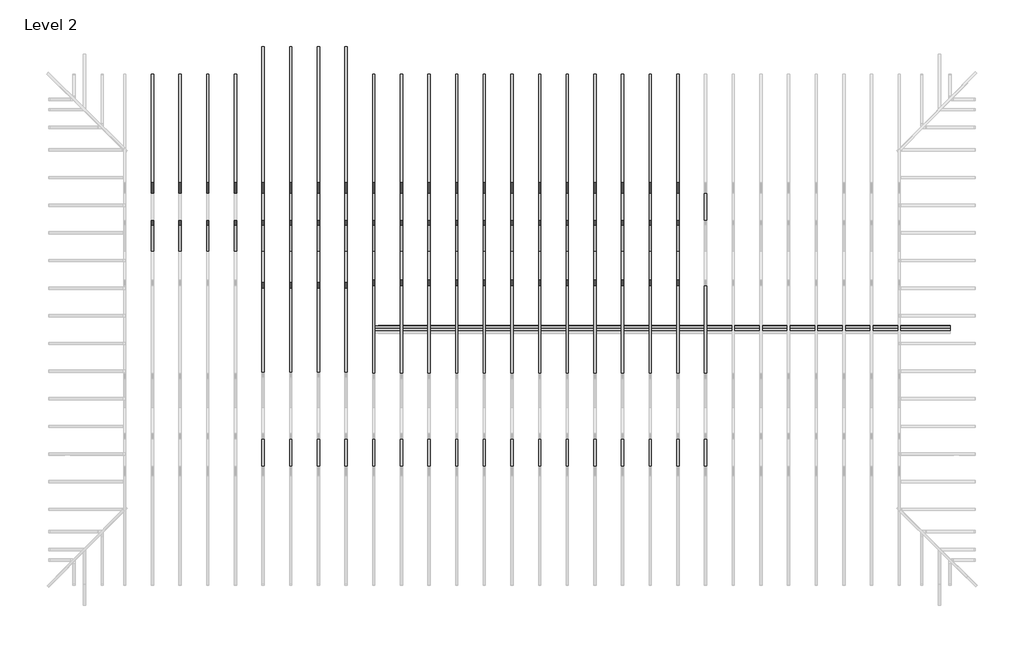
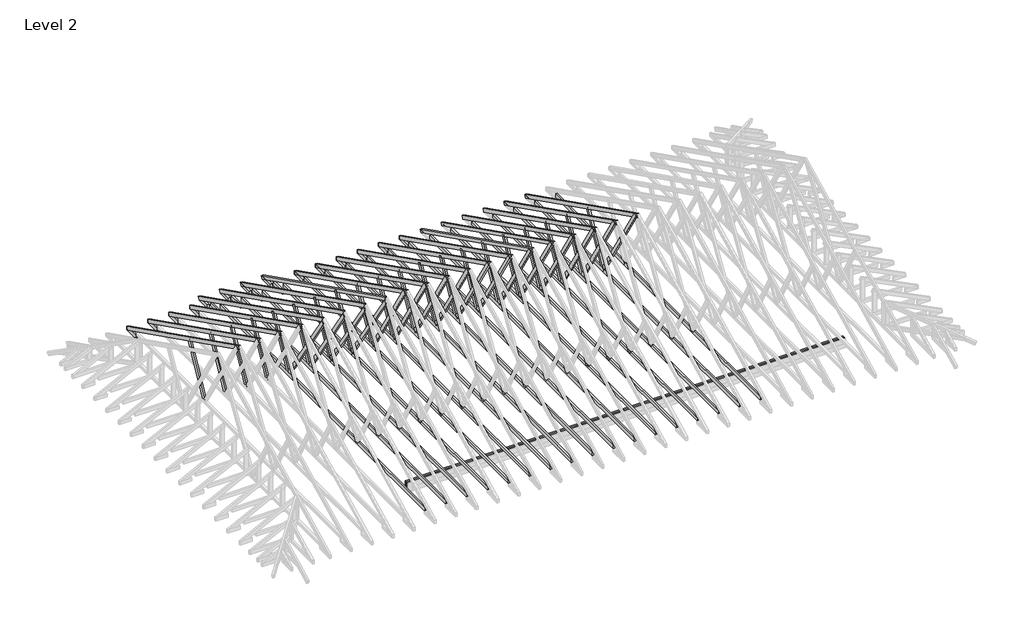
# One storey, part 4 of 5: 97 beams.
"""IFC4 building model written with IfcOpenShell, lengths in millimetres."""

import ifcopenshell
import ifcopenshell.guid

model = None  # the IFC model being written
_history = None  # IfcOwnerHistory: only IFC2X3 demands one
_inside = {}  # id of a spatial element -> (the spatial element, [elements in it])
_under = {}  # id of a project, library or spatial element -> (it, [spatial elements below it])
_declared = {}  # id of a project -> (the project, [libraries it declares])
_typed = {}  # id of a type object -> (the type object, [elements of that type])
_made_of = {}  # id of a material, layer set ... -> (it, [elements and type objects made of it])


def new_model(schema):
    """Start an empty IFC model of exactly this schema.

    Asked for "IFC4X3", IfcOpenShell would pick the latest addendum, in which some entities
    have other attributes; the version numbers below select the first issue.
    IFC2X3 requires an IfcOwnerHistory on every rooted entity: one is made here for all.
    """
    global model, _history
    if schema == "IFC4X3":
        model = ifcopenshell.file(schema_version=(4, 3, 0, 0))
    else:
        model = ifcopenshell.file(schema=schema)
    _inside.clear()
    _under.clear()
    _declared.clear()
    _typed.clear()
    _made_of.clear()
    _history = None
    if model.schema == "IFC2X3":
        org = make("IfcOrganization", Name="unknown")
        user = make(
            "IfcPersonAndOrganization",
            ThePerson=make("IfcPerson", FamilyName="unknown"),
            TheOrganization=org,
        )
        app = make(
            "IfcApplication",
            ApplicationDeveloper=org,
            Version="unknown",
            ApplicationFullName="unknown",
            ApplicationIdentifier="unknown",
        )
        _history = make(
            "IfcOwnerHistory",
            OwningUser=user,
            OwningApplication=app,
            ChangeAction="ADDED",
            CreationDate=0,
        )
    return model


def make(cls, **values):
    """One entity of the class cls with the attributes given. An attribute that is None is left unset."""
    return model.create_entity(
        cls, **{name: value for name, value in values.items() if value is not None}
    )


def rooted(cls, **values):
    """An entity with a GlobalId (a new one), such as an element, a storey or a relation."""
    return make(cls, GlobalId=ifcopenshell.guid.new(), OwnerHistory=_history, **values)


def si_unit(unit_type, name, prefix=None):
    """IfcSIUnit, for example si_unit("LENGTHUNIT", "METRE", prefix="MILLI")."""
    return make("IfcSIUnit", UnitType=unit_type, Prefix=prefix, Name=name)


def assignment(units):
    """IfcUnitAssignment: the units of a project."""
    return None if units is None else make("IfcUnitAssignment", Units=units)


def point(xyz):
    """IfcCartesianPoint."""
    return None if xyz is None else make("IfcCartesianPoint", Coordinates=xyz)


def direction(xyz):
    """IfcDirection."""
    return None if xyz is None else make("IfcDirection", DirectionRatios=xyz)


def frame(location, z_axis=None, x_axis=None):
    """IfcAxis2Placement3D, a coordinate frame: its origin and axes. An axis left out is left unset."""
    return make(
        "IfcAxis2Placement3D",
        Location=point(location),
        Axis=direction(z_axis),
        RefDirection=direction(x_axis),
    )


def origin():
    """The frame at (0, 0, 0) with its axes left unset."""
    return frame((0.0, 0.0, 0.0))


def place(relative_to, where):
    """IfcLocalPlacement: puts the frame where relative to a parent placement (None: the world)."""
    return make(
        "IfcLocalPlacement", PlacementRelTo=relative_to, RelativePlacement=where
    )


def context(
    kind, dimensions, precision=None, world=None, true_north=None, identifier=None
):
    """IfcGeometricRepresentationContext, for example the 3D "Model" context."""
    return make(
        "IfcGeometricRepresentationContext",
        ContextIdentifier=identifier,
        ContextType=kind,
        CoordinateSpaceDimension=dimensions,
        Precision=precision,
        WorldCoordinateSystem=world,
        TrueNorth=true_north,
    )


def project(units=None, contexts=None):
    """IfcProject with its units and contexts."""
    return rooted(
        "IfcProject",
        Name="project",
        RepresentationContexts=contexts,
        UnitsInContext=assignment(units),
    )


def spatial(cls, under=None, at=None, **own):
    """A site, building, storey or space (cls), placed at a placement, below another one or the project."""
    s = rooted(cls, ObjectPlacement=at, **own)
    if under is not None:
        _under.setdefault(under.id(), (under, []))[1].append(s)
    return s


def polyline(points):
    """IfcPolyline through the points."""
    return make("IfcPolyline", Points=[point(p) for p in points])


def outline(outer, holes=None, kind="AREA"):
    """IfcArbitraryClosedProfileDef: a profile drawn as a closed curve; with holes, ...WithVoids."""
    if holes is None:
        return make("IfcArbitraryClosedProfileDef", ProfileType=kind, OuterCurve=outer)
    return make(
        "IfcArbitraryProfileDefWithVoids",
        ProfileType=kind,
        OuterCurve=outer,
        InnerCurves=holes,
    )


def extrude(swept, where, along, depth):
    """IfcExtrudedAreaSolid: the profile swept, set in the frame where, extruded along a direction by depth."""
    return make(
        "IfcExtrudedAreaSolid",
        SweptArea=swept,
        Position=where,
        ExtrudedDirection=direction(along),
        Depth=depth,
    )


def shape(context_of_items, identifier, shape_type, items):
    """IfcShapeRepresentation: the items that make up one representation, for example the "Body"."""
    return make(
        "IfcShapeRepresentation",
        ContextOfItems=context_of_items,
        RepresentationIdentifier=identifier,
        RepresentationType=shape_type,
        Items=items,
    )


def source(mapping_origin, context_of_items, identifier, shape_type, items):
    """IfcRepresentationMap: a shape defined once, which mapped items show again and again."""
    return make(
        "IfcRepresentationMap",
        MappingOrigin=mapping_origin,
        MappedRepresentation=shape(context_of_items, identifier, shape_type, items),
    )


def transform(
    local_origin,
    x_axis=None,
    y_axis=None,
    z_axis=None,
    scale=None,
    scale2=None,
    scale3=None,
    uniform=True,
):
    """IfcCartesianTransformationOperator3D, or its non-uniform kind. x_axis, y_axis, z_axis: its Axis1, 2, 3."""
    if uniform:
        return make(
            "IfcCartesianTransformationOperator3D",
            Axis1=direction(x_axis),
            Axis2=direction(y_axis),
            LocalOrigin=point(local_origin),
            Scale=scale,
            Axis3=direction(z_axis),
        )
    return make(
        "IfcCartesianTransformationOperator3DnonUniform",
        Axis1=direction(x_axis),
        Axis2=direction(y_axis),
        LocalOrigin=point(local_origin),
        Scale=scale,
        Axis3=direction(z_axis),
        Scale2=scale2,
        Scale3=scale3,
    )


def mapped(mapping_source, mapping_target):
    """IfcMappedItem: shows the shape of a source again, moved by a transform."""
    return make(
        "IfcMappedItem", MappingSource=mapping_source, MappingTarget=mapping_target
    )


def made_of(thing, what):
    """Note that an element or type object is made of a material, layer set ...; save() writes the relation."""
    if what is not None:
        _made_of.setdefault(what.id(), (what, []))[1].append(thing)
    return thing


def element(
    cls,
    number,
    at=None,
    inside=None,
    cuts=None,
    type_object=None,
    material=None,
    context=None,
    identifier="Body",
    shape_type=None,
    held_by="IfcProductDefinitionShape",
    body=None,
    shapes=None,
    **own,
):
    """One element of the class cls, such as IfcWall. Its Tag is "e" and its number.

    at: its placement. inside: the storey or other place that contains it. cuts: it is an
    opening in that element (IfcRelVoidsElement). A single representation is given by context,
    identifier, shape_type and body (its items); several are given by shapes. held_by: the class
    of the entity that holds the representations. save() writes the other relations.
    """
    e = rooted(cls, Tag="e%d" % number, ObjectPlacement=at, **own)
    if body is not None:
        shapes = [shape(context, identifier, shape_type, body)]
    if shapes is not None:
        e.Representation = make(held_by, Representations=shapes)
    if inside is not None:
        _inside.setdefault(inside.id(), (inside, []))[1].append(e)
    if cuts is not None:
        rooted(
            "IfcRelVoidsElement", RelatingBuildingElement=cuts, RelatedOpeningElement=e
        )
    if type_object is not None:
        _typed.setdefault(type_object.id(), (type_object, []))[1].append(e)
    return made_of(e, material)


def aggregate(whole, parts):
    """IfcRelAggregates: a whole, such as a stair, and the parts it consists of."""
    return rooted("IfcRelAggregates", RelatingObject=whole, RelatedObjects=parts)


def save(model, path):
    """Write the relations noted so far, then the file.

    IfcRelAggregates (storeys below a building ...), IfcRelContainedInSpatialStructure (elements
    in a storey), IfcRelDefinesByType, IfcRelAssociatesMaterial and IfcRelDeclares: one each for
    every whole, place, type object, material and project.
    """
    for whole, parts in _under.values():
        aggregate(whole, parts)
    for where, things in _inside.values():
        rooted(
            "IfcRelContainedInSpatialStructure",
            RelatedElements=things,
            RelatingStructure=where,
        )
    for kind, things in _typed.values():
        rooted("IfcRelDefinesByType", RelatedObjects=things, RelatingType=kind)
    for what, things in _made_of.values():
        rooted("IfcRelAssociatesMaterial", RelatedObjects=things, RelatingMaterial=what)
    for by, libraries in _declared.values():
        rooted("IfcRelDeclares", RelatingContext=by, RelatedDefinitions=libraries)
    model.write(path)


def beam_b78a0881(model_context):
    return source(origin(), model_context, "Body", "SweptSolid", [
        extrude(outline(polyline([(228.6, 25.4), (228.6, -25.4), (-228.6, -25.4), (-228.6, 25.4), (228.6, 25.4)])), frame((0.0, 0.0, -50.8), z_axis=(0.0, 0.0, 1.0), x_axis=(1.0, 0.0, 0.0)), (0.0, 0.0, 1.0), 101.6),
    ])


def beam_90eea034(model_context):
    return source(origin(), model_context, "Body", "SweptSolid", [
        extrude(outline(polyline([(821.193698, 25.4), (821.193698, -25.4), (-819.5010489, -25.4), (-819.5010489, 25.4), (821.193698, 25.4)])), frame((0.0, 0.0, -50.8), z_axis=(0.0, 0.0, 1.0), x_axis=(1.0, 0.0, 0.0)), (0.0, 0.0, 1.0), 101.6),
    ])


def beam_a4242642(model_context):
    return source(origin(), model_context, "Body", "SweptSolid", [
        extrude(outline(polyline([(5145.3336481, 25.4), (5145.3336481, -25.4), (-5145.3336481, -25.4), (-5145.3336481, 25.4), (5145.3336481, 25.4)])), frame((0.0, 0.0, -50.8), z_axis=(0.0, 0.0, 1.0), x_axis=(1.0, 0.0, 0.0)), (0.0, 0.0, 1.0), 101.6),
    ])


def beam_fc8bf4ae(model_context):
    return source(origin(), model_context, "Body", "SweptSolid", [
        extrude(outline(polyline([(1562.6646551, 25.4), (1562.6646551, -25.4), (-1550.1468127, -25.4), (-1550.1468127, 25.4), (1562.6646551, 25.4)])), frame((0.0, 0.0, -50.8), z_axis=(0.0, 0.0, 1.0), x_axis=(1.0, 0.0, 0.0)), (0.0, 0.0, 1.0), 101.6),
    ])


def beam_2924e986(model_context):
    return source(origin(), model_context, "Body", "SweptSolid", [
        extrude(outline(polyline([(228.5999994, 25.4), (228.5999994, -25.4), (-179.8629717, -25.4), (-179.8629717, 25.4), (228.5999994, 25.4)])), frame((0.0, 0.0, -50.8), z_axis=(0.0, 0.0, 1.0), x_axis=(1.0, 0.0, 0.0)), (0.0, 0.0, 1.0), 101.6),
    ])


def beam_189f326c(model_context):
    return source(origin(), model_context, "Body", "SweptSolid", [
        extrude(outline(polyline([(1574.4380265, 25.4), (1574.4380265, -25.4), (-1601.4606477, -25.4), (-1601.4606477, 25.4), (1574.4380265, 25.4)])), frame((0.0, 0.0, -50.8), z_axis=(0.0, 0.0, 1.0), x_axis=(1.0, 0.0, 0.0)), (0.0, 0.0, 1.0), 101.6),
    ])


def beam_af7bd0b6(model_context):
    return source(origin(), model_context, "Body", "SweptSolid", [
        extrude(outline(polyline([(228.6, 25.4), (228.6, -25.4), (-179.8629717, -25.4), (-179.8629717, 25.4), (228.6, 25.4)])), frame((0.0, 0.0, -50.8), z_axis=(0.0, 0.0, 1.0), x_axis=(1.0, 0.0, 0.0)), (0.0, 0.0, 1.0), 101.6),
    ])


def beam_bcf194da(model_context):
    return source(origin(), model_context, "Body", "SweptSolid", [
        extrude(outline(polyline([(6302.375, 25.4), (6302.375, -25.4), (-6429.375, -25.4), (-6429.375, 25.4), (6302.375, 25.4)])), frame((0.0, 0.0, -127.0), z_axis=(0.0, 0.0, 1.0), x_axis=(1.0, 0.0, 0.0)), (0.0, 0.0, 1.0), 254.0),
    ])


def beam_af2566d3(model_context):
    return source(origin(), model_context, "Body", "SweptSolid", [
        extrude(outline(polyline([(6458.3020508, 5.55625), (6458.3020508, -5.55625), (-6159.1479492, -5.55625), (-6159.1479492, 5.55625), (6458.3020508, 5.55625)])), frame((0.0, 0.0, -63.5), z_axis=(0.0, 0.0, 1.0), x_axis=(1.0, 0.0, 0.0)), (0.0, 0.0, 1.0), 127.0),
    ])


model = new_model("IFC4")

# Units and contexts
model_context = context("Model", 3, world=origin())
ifc_project = project(units=[si_unit("LENGTHUNIT", "METRE", prefix="MILLI")], contexts=[model_context])

# Site, building, storey
site = spatial("IfcSite", under=ifc_project)
building = spatial("IfcBuilding", under=site)
storey = spatial("IfcBuildingStorey", under=building, Name="Level 2", Elevation=2768.6)

# Beams
placement = place(None, origin())
element("IfcBeam", 1, ObjectType="Dimension Lumber : BLDG 6241 2X4\" TRUSS MEMBER", at=placement, inside=storey, context=model_context, shape_type="SweptSolid", body=[
    extrude(outline(polyline([(0.0, -50.8), (0.0, 0.0), (6948.260151, 0.0), (6948.260151, -50.8), (0.0, -50.8)])), frame((-13559.414829, 10.7781069, 5482.082899), z_axis=(0.0, 0.4472135954999579, 0.894427190999916), x_axis=(0.0, 0.894427190999916, -0.4472135954999579)), (0.0, 0.0, 1.0), 101.6),
])
element("IfcBeam", 2, ObjectType="Dimension Lumber : BLDG 6241 2X4\" TRUSS MEMBER", at=placement, inside=storey, context=model_context, shape_type="SweptSolid", body=[
    extrude(outline(polyline([(0.0, -50.8), (0.0, 0.0), (6948.260151, 0.0), (6948.260151, -50.8), (0.0, -50.8)])), frame((-12949.814829, 10.7781069, 5482.082899), z_axis=(0.0, 0.44721359549995804, 0.894427190999916), x_axis=(0.0, 0.894427190999916, -0.44721359549995804)), (0.0, 0.0, 1.0), 101.6),
])
element("IfcBeam", 3, ObjectType="Dimension Lumber : BLDG 6241 2X4\" TRUSS MEMBER", at=placement, inside=storey, context=model_context, shape_type="SweptSolid", body=[
    extrude(outline(polyline([(0.0, -50.8), (0.0, 0.0), (6948.260151, 0.0), (6948.260151, -50.8), (0.0, -50.8)])), frame((-12340.214829, 10.7781069, 5482.082899), z_axis=(0.0, 0.44721359549995804, 0.894427190999916), x_axis=(0.0, 0.894427190999916, -0.44721359549995804)), (0.0, 0.0, 1.0), 101.6),
])
element("IfcBeam", 4, ObjectType="Dimension Lumber : BLDG 6241 2X4\" TRUSS MEMBER", at=placement, inside=storey, context=model_context, shape_type="SweptSolid", body=[
    extrude(outline(polyline([(0.0, -50.8), (0.0, 0.0), (6948.260151, 0.0), (6948.260151, -50.8), (0.0, -50.8)])), frame((-11730.614829, 10.7781069, 5482.082899), z_axis=(0.0, 0.44721359549995804, 0.894427190999916), x_axis=(0.0, 0.894427190999916, -0.44721359549995804)), (0.0, 0.0, 1.0), 101.6),
])
element("IfcBeam", 5, ObjectType="Dimension Lumber : BLDG 6241 2X4\" TRUSS MEMBER", at=placement, inside=storey, context=model_context, shape_type="SweptSolid", body=[
    extrude(outline(polyline([(0.0, -50.8), (0.0, 0.0), (6302.2496334, 0.0), (6302.2496334, -50.8), (0.0, -50.8)])), frame((-15997.814829, -17.2791662, 5496.1115355), z_axis=(0.0, 0.447213595499956, 0.894427190999917), x_axis=(0.0, 0.894427190999917, -0.447213595499956)), (0.0, 0.0, 1.0), 101.6),
])
element("IfcBeam", 6, ObjectType="Dimension Lumber : BLDG 6241 2X4\" TRUSS MEMBER", at=placement, inside=storey, context=model_context, shape_type="SweptSolid", body=[
    extrude(outline(polyline([(0.0, -50.8), (0.0, 0.0), (6302.2496334, 0.0), (6302.2496334, -50.8), (0.0, -50.8)])), frame((-15388.214829, -17.2791662, 5496.1115355), z_axis=(0.0, 0.447213595499956, 0.894427190999917), x_axis=(0.0, 0.894427190999917, -0.447213595499956)), (0.0, 0.0, 1.0), 101.6),
])
element("IfcBeam", 7, ObjectType="Dimension Lumber : BLDG 6241 2X4\" TRUSS MEMBER", at=placement, inside=storey, context=model_context, shape_type="SweptSolid", body=[
    extrude(outline(polyline([(0.0, -50.8), (0.0, 0.0), (6302.2496334, 0.0), (6302.2496334, -50.8), (0.0, -50.8)])), frame((-14778.614829, -17.2791662, 5496.1115355), z_axis=(0.0, 0.44721359549995576, 0.8944271909999171), x_axis=(0.0, 0.8944271909999171, -0.44721359549995576)), (0.0, 0.0, 1.0), 101.6),
])
element("IfcBeam", 8, ObjectType="Dimension Lumber : BLDG 6241 2X4\" TRUSS MEMBER", at=placement, inside=storey, context=model_context, shape_type="SweptSolid", body=[
    extrude(outline(polyline([(0.0, -50.8), (0.0, 0.0), (6302.2496334, 0.0), (6302.2496334, -50.8), (0.0, -50.8)])), frame((-14169.014829, -17.2791662, 5496.1115355), z_axis=(0.0, 0.447213595499956, 0.894427190999917), x_axis=(0.0, 0.894427190999917, -0.447213595499956)), (0.0, 0.0, 1.0), 101.6),
])
element("IfcBeam", 9, ObjectType="Dimension Lumber : BLDG 6241 2X4\" TRUSS MEMBER", at=placement, inside=storey, context=model_context, shape_type="SweptSolid", body=[
    extrude(outline(polyline([(0.0, -50.8), (0.0, 0.0), (6302.2496334, 0.0), (6302.2496334, -50.8), (0.0, -50.8)])), frame((-11121.014829, -17.2791662, 5496.1115355), z_axis=(0.0, 0.447213595499956, 0.894427190999917), x_axis=(0.0, 0.894427190999917, -0.447213595499956)), (0.0, 0.0, 1.0), 101.6),
])
element("IfcBeam", 10, ObjectType="Dimension Lumber : BLDG 6241 2X4\" TRUSS MEMBER", at=placement, inside=storey, context=model_context, shape_type="SweptSolid", body=[
    extrude(outline(polyline([(0.0, -50.8), (0.0, 0.0), (6302.2496334, 0.0), (6302.2496334, -50.8), (0.0, -50.8)])), frame((-10511.414829, -17.2791662, 5496.1115355), z_axis=(0.0, 0.4472135954999559, 0.894427190999917), x_axis=(0.0, 0.894427190999917, -0.4472135954999559)), (0.0, 0.0, 1.0), 101.6),
])
element("IfcBeam", 11, ObjectType="Dimension Lumber : BLDG 6241 2X4\" TRUSS MEMBER", at=placement, inside=storey, context=model_context, shape_type="SweptSolid", body=[
    extrude(outline(polyline([(0.0, -50.8), (0.0, 0.0), (6302.2496334, 0.0), (6302.2496334, -50.8), (0.0, -50.8)])), frame((-9901.814829, -17.2791662, 5496.1115355), z_axis=(0.0, 0.44721359549995576, 0.894427190999917), x_axis=(0.0, 0.894427190999917, -0.44721359549995576)), (0.0, 0.0, 1.0), 101.6),
])
element("IfcBeam", 12, ObjectType="Dimension Lumber : BLDG 6241 2X4\" TRUSS MEMBER", at=placement, inside=storey, context=model_context, shape_type="SweptSolid", body=[
    extrude(outline(polyline([(0.0, -50.8), (0.0, 0.0), (6302.2496334, 0.0), (6302.2496334, -50.8), (0.0, -50.8)])), frame((-9292.214829, -17.2791662, 5496.1115355), z_axis=(0.0, 0.447213595499956, 0.8944271909999169), x_axis=(0.0, 0.8944271909999169, -0.447213595499956)), (0.0, 0.0, 1.0), 101.6),
])
element("IfcBeam", 13, ObjectType="Dimension Lumber : BLDG 6241 2X4\" TRUSS MEMBER", at=placement, inside=storey, context=model_context, shape_type="SweptSolid", body=[
    extrude(outline(polyline([(0.0, -50.8), (0.0, 0.0), (6302.2496334, 0.0), (6302.2496334, -50.8), (0.0, -50.8)])), frame((-8682.614829, -17.2791662, 5496.1115355), z_axis=(0.0, 0.44721359549995593, 0.894427190999917), x_axis=(0.0, 0.894427190999917, -0.44721359549995593)), (0.0, 0.0, 1.0), 101.6),
])
element("IfcBeam", 14, ObjectType="Dimension Lumber : BLDG 6241 2X4\" TRUSS MEMBER", at=placement, inside=storey, context=model_context, shape_type="SweptSolid", body=[
    extrude(outline(polyline([(0.0, -50.8), (0.0, 0.0), (6302.2496334, 0.0), (6302.2496334, -50.8), (0.0, -50.8)])), frame((-8073.014829, -17.2791662, 5496.1115355), z_axis=(0.0, 0.4472135954999558, 0.894427190999917), x_axis=(0.0, 0.894427190999917, -0.4472135954999558)), (0.0, 0.0, 1.0), 101.6),
])
element("IfcBeam", 15, ObjectType="Dimension Lumber : BLDG 6241 2X4\" TRUSS MEMBER", at=placement, inside=storey, context=model_context, shape_type="SweptSolid", body=[
    extrude(outline(polyline([(0.0, -50.8), (0.0, 0.0), (6302.2496334, 0.0), (6302.2496334, -50.8), (0.0, -50.8)])), frame((-7463.414829, -17.2791662, 5496.1115355), z_axis=(0.0, 0.4472135954999557, 0.894427190999917), x_axis=(0.0, 0.894427190999917, -0.4472135954999557)), (0.0, 0.0, 1.0), 101.6),
])
element("IfcBeam", 16, ObjectType="Dimension Lumber : BLDG 6241 2X4\" TRUSS MEMBER", at=placement, inside=storey, context=model_context, shape_type="SweptSolid", body=[
    extrude(outline(polyline([(0.0, -50.8), (0.0, 0.0), (6302.2496334, 0.0), (6302.2496334, -50.8), (0.0, -50.8)])), frame((-6853.814829, -17.2791662, 5496.1115355), z_axis=(0.0, 0.4472135954999561, 0.8944271909999169), x_axis=(0.0, 0.8944271909999169, -0.4472135954999561)), (0.0, 0.0, 1.0), 101.6),
])
element("IfcBeam", 17, ObjectType="Dimension Lumber : BLDG 6241 2X4\" TRUSS MEMBER", at=placement, inside=storey, context=model_context, shape_type="SweptSolid", body=[
    extrude(outline(polyline([(0.0, -50.8), (0.0, 0.0), (6302.2496334, 0.0), (6302.2496334, -50.8), (0.0, -50.8)])), frame((-6244.214829, -17.2791662, 5496.1115355), z_axis=(0.0, 0.44721359549995593, 0.894427190999917), x_axis=(0.0, 0.894427190999917, -0.44721359549995593)), (0.0, 0.0, 1.0), 101.6),
])
element("IfcBeam", 18, ObjectType="Dimension Lumber : BLDG 6241 2X4\" TRUSS MEMBER", at=placement, inside=storey, context=model_context, shape_type="SweptSolid", body=[
    extrude(outline(polyline([(0.0, -50.8), (0.0, 0.0), (6302.2496334, 0.0), (6302.2496334, -50.8), (0.0, -50.8)])), frame((-5634.614829, -17.2791662, 5496.1115355), z_axis=(0.0, 0.447213595499956, 0.8944271909999169), x_axis=(0.0, 0.8944271909999169, -0.447213595499956)), (0.0, 0.0, 1.0), 101.6),
])
element("IfcBeam", 19, ObjectType="Dimension Lumber : BLDG 6241 2X4\" TRUSS MEMBER", at=placement, inside=storey, context=model_context, shape_type="SweptSolid", body=[
    extrude(outline(polyline([(0.0, -50.8), (0.0, 0.0), (6302.2496334, 0.0), (6302.2496334, -50.8), (0.0, -50.8)])), frame((-5025.014829, -17.2791662, 5496.1115355), z_axis=(0.0, 0.44721359549995593, 0.894427190999917), x_axis=(0.0, 0.894427190999917, -0.44721359549995593)), (0.0, 0.0, 1.0), 101.6),
])
element("IfcBeam", 20, ObjectType="Dimension Lumber : BLDG 6241 2X4\" TRUSS MEMBER", at=placement, inside=storey, context=model_context, shape_type="SweptSolid", body=[
    extrude(outline(polyline([(0.0, -50.8), (0.0, 0.0), (6302.2496334, 0.0), (6302.2496334, -50.8), (0.0, -50.8)])), frame((-4415.414829, -17.2791662, 5496.1115355), z_axis=(0.0, 0.4472135954999558, 0.894427190999917), x_axis=(0.0, 0.894427190999917, -0.4472135954999558)), (0.0, 0.0, 1.0), 101.6),
])
beam_shape = beam_b78a0881(model_context)
element("IfcBeam", 21, ObjectType="Dimension Lumber : BLDG 6241 2X4\" TRUSS MEMBER", at=placement, inside=storey, context=model_context, shape_type="MappedRepresentation", body=[
    mapped(beam_shape, transform((-13534.014829, 5436.3284114, 2589.5072623), x_axis=(0.0, -1.0, 0.0), y_axis=(1.0, 0.0, 0.0), z_axis=(0.0, 0.0, 1.0))),
])
element("IfcBeam", 22, ObjectType="Dimension Lumber : BLDG 6241 2X4\" TRUSS MEMBER", at=placement, inside=storey, context=model_context, shape_type="MappedRepresentation", body=[
    mapped(beam_shape, transform((-12924.414829, 5436.3284114, 2589.5072623), x_axis=(0.0, -1.0, 0.0), y_axis=(1.0, 0.0, 0.0), z_axis=(0.0, 0.0, 1.0))),
])
element("IfcBeam", 23, ObjectType="Dimension Lumber : BLDG 6241 2X4\" TRUSS MEMBER", at=placement, inside=storey, context=model_context, shape_type="MappedRepresentation", body=[
    mapped(beam_shape, transform((-12314.814829, 5436.3284114, 2589.5072623), x_axis=(0.0, -1.0, 0.0), y_axis=(1.0, 0.0, 0.0), z_axis=(0.0, 0.0, 1.0))),
])
element("IfcBeam", 24, ObjectType="Dimension Lumber : BLDG 6241 2X4\" TRUSS MEMBER", at=placement, inside=storey, context=model_context, shape_type="MappedRepresentation", body=[
    mapped(beam_shape, transform((-11705.214829, 5436.3284114, 2589.5072623), x_axis=(0.0, -1.0, 0.0), y_axis=(1.0, 0.0, 0.0), z_axis=(0.0, 0.0, 1.0))),
])
element("IfcBeam", 25, ObjectType="Dimension Lumber : BLDG 6241 2X4\" TRUSS MEMBER", at=placement, inside=storey, context=model_context, shape_type="MappedRepresentation", body=[
    mapped(beam_shape, transform((-12924.414829, 5436.3284114, 2589.5072623), x_axis=(0.0, -1.0, 0.0), y_axis=(1.0, 0.0, 0.0), z_axis=(0.0, 0.0, 1.0))),
])
element("IfcBeam", 26, ObjectType="Dimension Lumber : BLDG 6241 2X4\" TRUSS MEMBER", at=placement, inside=storey, context=model_context, shape_type="MappedRepresentation", body=[
    mapped(beam_shape, transform((-12314.814829, 5436.3284114, 2589.5072623), x_axis=(0.0, -1.0, 0.0), y_axis=(1.0, 0.0, 0.0), z_axis=(0.0, 0.0, 1.0))),
])
element("IfcBeam", 27, ObjectType="Dimension Lumber : BLDG 6241 2X4\" TRUSS MEMBER", at=placement, inside=storey, context=model_context, shape_type="MappedRepresentation", body=[
    mapped(beam_shape, transform((-11705.214829, 5436.3284114, 2589.5072623), x_axis=(0.0, -1.0, 0.0), y_axis=(1.0, 0.0, 0.0), z_axis=(0.0, 0.0, 1.0))),
])
element("IfcBeam", 28, ObjectType="Dimension Lumber : BLDG 6241 2X4\" TRUSS MEMBER", at=placement, inside=storey, context=model_context, shape_type="MappedRepresentation", body=[
    mapped(beam_shape, transform((-15972.414829, 5436.3284114, 2717.8), x_axis=(0.0, -1.0, 0.0), y_axis=(1.0, 0.0, 0.0), z_axis=(0.0, 0.0, 1.0))),
])
element("IfcBeam", 29, ObjectType="Dimension Lumber : BLDG 6241 2X4\" TRUSS MEMBER", at=placement, inside=storey, context=model_context, shape_type="MappedRepresentation", body=[
    mapped(beam_shape, transform((-15362.814829, 5436.3284114, 2717.8), x_axis=(0.0, -1.0, 0.0), y_axis=(1.0, 0.0, 0.0), z_axis=(0.0, 0.0, 1.0))),
])
element("IfcBeam", 30, ObjectType="Dimension Lumber : BLDG 6241 2X4\" TRUSS MEMBER", at=placement, inside=storey, context=model_context, shape_type="MappedRepresentation", body=[
    mapped(beam_shape, transform((-14753.214829, 5436.3284114, 2717.8), x_axis=(0.0, -1.0, 0.0), y_axis=(1.0, 0.0, 0.0), z_axis=(0.0, 0.0, 1.0))),
])
element("IfcBeam", 31, ObjectType="Dimension Lumber : BLDG 6241 2X4\" TRUSS MEMBER", at=placement, inside=storey, context=model_context, shape_type="MappedRepresentation", body=[
    mapped(beam_shape, transform((-14143.614829, 5436.3284114, 2717.8), x_axis=(0.0, -1.0, 0.0), y_axis=(1.0, 0.0, 0.0), z_axis=(0.0, 0.0, 1.0))),
])
element("IfcBeam", 32, ObjectType="Dimension Lumber : BLDG 6241 2X4\" TRUSS MEMBER", at=placement, inside=storey, context=model_context, shape_type="MappedRepresentation", body=[
    mapped(beam_shape, transform((-11095.614829, 5436.3284114, 2717.8), x_axis=(0.0, -1.0, 0.0), y_axis=(1.0, 0.0, 0.0), z_axis=(0.0, 0.0, 1.0))),
])
element("IfcBeam", 33, ObjectType="Dimension Lumber : BLDG 6241 2X4\" TRUSS MEMBER", at=placement, inside=storey, context=model_context, shape_type="MappedRepresentation", body=[
    mapped(beam_shape, transform((-10486.014829, 5436.3284114, 2717.8), x_axis=(0.0, -1.0, 0.0), y_axis=(1.0, 0.0, 0.0), z_axis=(0.0, 0.0, 1.0))),
])
element("IfcBeam", 34, ObjectType="Dimension Lumber : BLDG 6241 2X4\" TRUSS MEMBER", at=placement, inside=storey, context=model_context, shape_type="MappedRepresentation", body=[
    mapped(beam_shape, transform((-9876.414829, 5436.3284114, 2717.8), x_axis=(0.0, -1.0, 0.0), y_axis=(1.0, 0.0, 0.0), z_axis=(0.0, 0.0, 1.0))),
])
element("IfcBeam", 35, ObjectType="Dimension Lumber : BLDG 6241 2X4\" TRUSS MEMBER", at=placement, inside=storey, context=model_context, shape_type="MappedRepresentation", body=[
    mapped(beam_shape, transform((-9266.814829, 5436.3284114, 2717.8), x_axis=(0.0, -1.0, 0.0), y_axis=(1.0, 0.0, 0.0), z_axis=(0.0, 0.0, 1.0))),
])
element("IfcBeam", 36, ObjectType="Dimension Lumber : BLDG 6241 2X4\" TRUSS MEMBER", at=placement, inside=storey, context=model_context, shape_type="MappedRepresentation", body=[
    mapped(beam_shape, transform((-8657.214829, 5436.3284114, 2717.8), x_axis=(0.0, -1.0, 0.0), y_axis=(1.0, 0.0, 0.0), z_axis=(0.0, 0.0, 1.0))),
])
element("IfcBeam", 37, ObjectType="Dimension Lumber : BLDG 6241 2X4\" TRUSS MEMBER", at=placement, inside=storey, context=model_context, shape_type="MappedRepresentation", body=[
    mapped(beam_shape, transform((-8047.614829, 5436.3284114, 2717.8), x_axis=(0.0, -1.0, 0.0), y_axis=(1.0, 0.0, 0.0), z_axis=(0.0, 0.0, 1.0))),
])
beam_2_shape = beam_90eea034(model_context)
element("IfcBeam", 38, ObjectType="Dimension Lumber : BLDG 6241 2X4\" TRUSS MEMBER", at=placement, inside=storey, context=model_context, shape_type="MappedRepresentation", body=[
    mapped(beam_2_shape, transform((-13534.014829, 2147.8781861, 3552.5770493), x_axis=(0.0, -0.48031726308520883, -0.87709482200178), y_axis=(-1.0, 0.0, 0.0), z_axis=(0.0, 0.87709482200178, -0.48031726308520883))),
])
element("IfcBeam", 39, ObjectType="Dimension Lumber : BLDG 6241 2X4\" TRUSS MEMBER", at=placement, inside=storey, context=model_context, shape_type="MappedRepresentation", body=[
    mapped(beam_2_shape, transform((-12924.414829, 2147.8781861, 3552.5770493), x_axis=(0.0, -0.48031726308520883, -0.87709482200178), y_axis=(-1.0, 0.0, 0.0), z_axis=(0.0, 0.87709482200178, -0.48031726308520883))),
])
element("IfcBeam", 40, ObjectType="Dimension Lumber : BLDG 6241 2X4\" TRUSS MEMBER", at=placement, inside=storey, context=model_context, shape_type="MappedRepresentation", body=[
    mapped(beam_2_shape, transform((-12314.814829, 2147.8781861, 3552.5770493), x_axis=(0.0, -0.48031726308520883, -0.87709482200178), y_axis=(-1.0, 0.0, 0.0), z_axis=(0.0, 0.87709482200178, -0.48031726308520883))),
])
element("IfcBeam", 41, ObjectType="Dimension Lumber : BLDG 6241 2X4\" TRUSS MEMBER", at=placement, inside=storey, context=model_context, shape_type="MappedRepresentation", body=[
    mapped(beam_2_shape, transform((-11705.214829, 2147.8781861, 3552.5770493), x_axis=(0.0, -0.48031726308520883, -0.87709482200178), y_axis=(-1.0, 0.0, 0.0), z_axis=(0.0, 0.87709482200178, -0.48031726308520883))),
])
element("IfcBeam", 42, ObjectType="Dimension Lumber : BLDG 6241 2X4\" TRUSS MEMBER", at=placement, inside=storey, context=model_context, shape_type="MappedRepresentation", body=[
    mapped(beam_2_shape, transform((-15972.414829, 2147.8781861, 3552.5770493), x_axis=(0.0, -0.4803172630852004, -0.8770948220017847), y_axis=(-1.0, 0.0, 0.0), z_axis=(0.0, 0.8770948220017847, -0.4803172630852004))),
])
element("IfcBeam", 43, ObjectType="Dimension Lumber : BLDG 6241 2X4\" TRUSS MEMBER", at=placement, inside=storey, context=model_context, shape_type="MappedRepresentation", body=[
    mapped(beam_2_shape, transform((-15362.814829, 2147.8781861, 3552.5770493), x_axis=(0.0, -0.4803172630852004, -0.8770948220017847), y_axis=(-1.0, 0.0, 0.0), z_axis=(0.0, 0.8770948220017847, -0.4803172630852004))),
])
element("IfcBeam", 44, ObjectType="Dimension Lumber : BLDG 6241 2X4\" TRUSS MEMBER", at=placement, inside=storey, context=model_context, shape_type="MappedRepresentation", body=[
    mapped(beam_2_shape, transform((-14753.214829, 2147.8781861, 3552.5770493), x_axis=(0.0, -0.4803172630852004, -0.8770948220017847), y_axis=(-1.0, 0.0, 0.0), z_axis=(0.0, 0.8770948220017847, -0.4803172630852004))),
])
element("IfcBeam", 45, ObjectType="Dimension Lumber : BLDG 6241 2X4\" TRUSS MEMBER", at=placement, inside=storey, context=model_context, shape_type="MappedRepresentation", body=[
    mapped(beam_2_shape, transform((-14143.614829, 2147.8781861, 3552.5770493), x_axis=(0.0, -0.4803172630852004, -0.8770948220017847), y_axis=(-1.0, 0.0, 0.0), z_axis=(0.0, 0.8770948220017847, -0.4803172630852004))),
])
element("IfcBeam", 46, ObjectType="Dimension Lumber : BLDG 6241 2X4\" TRUSS MEMBER", at=placement, inside=storey, context=model_context, shape_type="MappedRepresentation", body=[
    mapped(beam_2_shape, transform((-11095.614829, 2147.8781861, 3552.5770493), x_axis=(0.0, -0.4803172630852004, -0.8770948220017847), y_axis=(-1.0, 0.0, 0.0), z_axis=(0.0, 0.8770948220017847, -0.4803172630852004))),
])
element("IfcBeam", 47, ObjectType="Dimension Lumber : BLDG 6241 2X4\" TRUSS MEMBER", at=placement, inside=storey, context=model_context, shape_type="MappedRepresentation", body=[
    mapped(beam_2_shape, transform((-10486.014829, 2147.8781861, 3552.5770493), x_axis=(0.0, -0.4803172630852004, -0.8770948220017847), y_axis=(-1.0, 0.0, 0.0), z_axis=(0.0, 0.8770948220017847, -0.4803172630852004))),
])
element("IfcBeam", 48, ObjectType="Dimension Lumber : BLDG 6241 2X4\" TRUSS MEMBER", at=placement, inside=storey, context=model_context, shape_type="MappedRepresentation", body=[
    mapped(beam_2_shape, transform((-9876.414829, 2147.8781861, 3552.5770493), x_axis=(0.0, -0.4803172630852004, -0.8770948220017847), y_axis=(-1.0, 0.0, 0.0), z_axis=(0.0, 0.8770948220017847, -0.4803172630852004))),
])
element("IfcBeam", 49, ObjectType="Dimension Lumber : BLDG 6241 2X4\" TRUSS MEMBER", at=placement, inside=storey, context=model_context, shape_type="MappedRepresentation", body=[
    mapped(beam_2_shape, transform((-9266.814829, 2147.8781861, 3552.5770493), x_axis=(0.0, -0.4803172630852004, -0.8770948220017847), y_axis=(-1.0, 0.0, 0.0), z_axis=(0.0, 0.8770948220017847, -0.4803172630852004))),
])
element("IfcBeam", 50, ObjectType="Dimension Lumber : BLDG 6241 2X4\" TRUSS MEMBER", at=placement, inside=storey, context=model_context, shape_type="MappedRepresentation", body=[
    mapped(beam_2_shape, transform((-8657.214829, 2147.8781861, 3552.5770493), x_axis=(0.0, -0.4803172630852004, -0.8770948220017847), y_axis=(-1.0, 0.0, 0.0), z_axis=(0.0, 0.8770948220017847, -0.4803172630852004))),
])
element("IfcBeam", 51, ObjectType="Dimension Lumber : BLDG 6241 2X4\" TRUSS MEMBER", at=placement, inside=storey, context=model_context, shape_type="MappedRepresentation", body=[
    mapped(beam_2_shape, transform((-8047.614829, 2147.8781861, 3552.5770493), x_axis=(0.0, -0.4803172630852004, -0.8770948220017847), y_axis=(-1.0, 0.0, 0.0), z_axis=(0.0, 0.8770948220017847, -0.4803172630852004))),
])
element("IfcBeam", 52, ObjectType="Dimension Lumber : BLDG 6241 2X4\" TRUSS MEMBER", at=placement, inside=storey, context=model_context, shape_type="MappedRepresentation", body=[
    mapped(beam_2_shape, transform((-7438.014829, 2147.8781861, 3552.5770493), x_axis=(0.0, -0.4803172630852004, -0.8770948220017847), y_axis=(-1.0, 0.0, 0.0), z_axis=(0.0, 0.8770948220017847, -0.4803172630852004))),
])
element("IfcBeam", 53, ObjectType="Dimension Lumber : BLDG 6241 2X4\" TRUSS MEMBER", at=placement, inside=storey, context=model_context, shape_type="MappedRepresentation", body=[
    mapped(beam_2_shape, transform((-6828.414829, 2147.8781861, 3552.5770493), x_axis=(0.0, -0.4803172630852004, -0.8770948220017847), y_axis=(-1.0, 0.0, 0.0), z_axis=(0.0, 0.8770948220017847, -0.4803172630852004))),
])
element("IfcBeam", 54, ObjectType="Dimension Lumber : BLDG 6241 2X4\" TRUSS MEMBER", at=placement, inside=storey, context=model_context, shape_type="MappedRepresentation", body=[
    mapped(beam_2_shape, transform((-6218.814829, 2147.8781861, 3552.5770493), x_axis=(0.0, -0.4803172630852004, -0.8770948220017847), y_axis=(-1.0, 0.0, 0.0), z_axis=(0.0, 0.8770948220017847, -0.4803172630852004))),
])
element("IfcBeam", 55, ObjectType="Dimension Lumber : BLDG 6241 2X4\" TRUSS MEMBER", at=placement, inside=storey, context=model_context, shape_type="MappedRepresentation", body=[
    mapped(beam_2_shape, transform((-5609.214829, 2147.8781861, 3552.5770493), x_axis=(0.0, -0.4803172630852004, -0.8770948220017847), y_axis=(-1.0, 0.0, 0.0), z_axis=(0.0, 0.8770948220017847, -0.4803172630852004))),
])
element("IfcBeam", 56, ObjectType="Dimension Lumber : BLDG 6241 2X4\" TRUSS MEMBER", at=placement, inside=storey, context=model_context, shape_type="MappedRepresentation", body=[
    mapped(beam_2_shape, transform((-4999.614829, 2147.8781861, 3552.5770493), x_axis=(0.0, -0.4803172630852004, -0.8770948220017847), y_axis=(-1.0, 0.0, 0.0), z_axis=(0.0, 0.8770948220017847, -0.4803172630852004))),
])
element("IfcBeam", 57, ObjectType="Dimension Lumber : BLDG 6241 2X4\" TRUSS MEMBER", at=placement, inside=storey, context=model_context, shape_type="MappedRepresentation", body=[
    mapped(beam_2_shape, transform((-4390.014829, 2147.8781861, 3552.5770493), x_axis=(0.0, -0.4803172630852004, -0.8770948220017847), y_axis=(-1.0, 0.0, 0.0), z_axis=(0.0, 0.8770948220017847, -0.4803172630852004))),
])
beam_3_shape = beam_a4242642(model_context)
element("IfcBeam", 58, ObjectType="Dimension Lumber : BLDG 6241 2X4\" TRUSS MEMBER", at=placement, inside=storey, context=model_context, shape_type="MappedRepresentation", body=[
    mapped(beam_3_shape, transform((-13534.014829, 26.1284114, 2819.4), x_axis=(0.0, -1.0, 0.0), y_axis=(1.0, 0.0, 0.0), z_axis=(0.0, 0.0, 1.0))),
])
element("IfcBeam", 59, ObjectType="Dimension Lumber : BLDG 6241 2X4\" TRUSS MEMBER", at=placement, inside=storey, context=model_context, shape_type="MappedRepresentation", body=[
    mapped(beam_3_shape, transform((-12924.414829, 26.1284114, 2819.4), x_axis=(0.0, -1.0, 0.0), y_axis=(1.0, 0.0, 0.0), z_axis=(0.0, 0.0, 1.0))),
])
element("IfcBeam", 60, ObjectType="Dimension Lumber : BLDG 6241 2X4\" TRUSS MEMBER", at=placement, inside=storey, context=model_context, shape_type="MappedRepresentation", body=[
    mapped(beam_3_shape, transform((-12314.814829, 26.1284114, 2819.4), x_axis=(0.0, -1.0, 0.0), y_axis=(1.0, 0.0, 0.0), z_axis=(0.0, 0.0, 1.0))),
])
element("IfcBeam", 61, ObjectType="Dimension Lumber : BLDG 6241 2X4\" TRUSS MEMBER", at=placement, inside=storey, context=model_context, shape_type="MappedRepresentation", body=[
    mapped(beam_3_shape, transform((-11705.214829, 26.1284114, 2819.4), x_axis=(0.0, -1.0, 0.0), y_axis=(1.0, 0.0, 0.0), z_axis=(0.0, 0.0, 1.0))),
])
element("IfcBeam", 62, ObjectType="Dimension Lumber : BLDG 6241 2X4\" TRUSS MEMBER", at=placement, inside=storey, context=model_context, shape_type="MappedRepresentation", body=[
    mapped(beam_3_shape, transform((-11095.614829, 26.1284114, 2819.4), x_axis=(0.0, -1.0, 0.0), y_axis=(1.0, 0.0, 0.0), z_axis=(0.0, 0.0, 1.0))),
])
element("IfcBeam", 63, ObjectType="Dimension Lumber : BLDG 6241 2X4\" TRUSS MEMBER", at=placement, inside=storey, context=model_context, shape_type="MappedRepresentation", body=[
    mapped(beam_3_shape, transform((-10486.014829, 26.1284114, 2819.4), x_axis=(0.0, -1.0, 0.0), y_axis=(1.0, 0.0, 0.0), z_axis=(0.0, 0.0, 1.0))),
])
element("IfcBeam", 64, ObjectType="Dimension Lumber : BLDG 6241 2X4\" TRUSS MEMBER", at=placement, inside=storey, context=model_context, shape_type="MappedRepresentation", body=[
    mapped(beam_3_shape, transform((-9876.414829, 26.1284114, 2819.4), x_axis=(0.0, -1.0, 0.0), y_axis=(1.0, 0.0, 0.0), z_axis=(0.0, 0.0, 1.0))),
])
element("IfcBeam", 65, ObjectType="Dimension Lumber : BLDG 6241 2X4\" TRUSS MEMBER", at=placement, inside=storey, context=model_context, shape_type="MappedRepresentation", body=[
    mapped(beam_3_shape, transform((-9266.814829, 26.1284114, 2819.4), x_axis=(0.0, -1.0, 0.0), y_axis=(1.0, 0.0, 0.0), z_axis=(0.0, 0.0, 1.0))),
])
element("IfcBeam", 66, ObjectType="Dimension Lumber : BLDG 6241 2X4\" TRUSS MEMBER", at=placement, inside=storey, context=model_context, shape_type="MappedRepresentation", body=[
    mapped(beam_3_shape, transform((-8657.214829, 26.1284114, 2819.4), x_axis=(0.0, -1.0, 0.0), y_axis=(1.0, 0.0, 0.0), z_axis=(0.0, 0.0, 1.0))),
])
element("IfcBeam", 67, ObjectType="Dimension Lumber : BLDG 6241 2X4\" TRUSS MEMBER", at=placement, inside=storey, context=model_context, shape_type="MappedRepresentation", body=[
    mapped(beam_3_shape, transform((-8047.614829, 26.1284114, 2819.4), x_axis=(0.0, -1.0, 0.0), y_axis=(1.0, 0.0, 0.0), z_axis=(0.0, 0.0, 1.0))),
])
element("IfcBeam", 68, ObjectType="Dimension Lumber : BLDG 6241 2X4\" TRUSS MEMBER", at=placement, inside=storey, context=model_context, shape_type="MappedRepresentation", body=[
    mapped(beam_3_shape, transform((-7438.014829, 26.1284114, 2819.4), x_axis=(0.0, -1.0, 0.0), y_axis=(1.0, 0.0, 0.0), z_axis=(0.0, 0.0, 1.0))),
])
element("IfcBeam", 69, ObjectType="Dimension Lumber : BLDG 6241 2X4\" TRUSS MEMBER", at=placement, inside=storey, context=model_context, shape_type="MappedRepresentation", body=[
    mapped(beam_3_shape, transform((-6828.414829, 26.1284114, 2819.4), x_axis=(0.0, -1.0, 0.0), y_axis=(1.0, 0.0, 0.0), z_axis=(0.0, 0.0, 1.0))),
])
element("IfcBeam", 70, ObjectType="Dimension Lumber : BLDG 6241 2X4\" TRUSS MEMBER", at=placement, inside=storey, context=model_context, shape_type="MappedRepresentation", body=[
    mapped(beam_3_shape, transform((-6218.814829, 26.1284114, 2819.4), x_axis=(0.0, -1.0, 0.0), y_axis=(1.0, 0.0, 0.0), z_axis=(0.0, 0.0, 1.0))),
])
element("IfcBeam", 71, ObjectType="Dimension Lumber : BLDG 6241 2X4\" TRUSS MEMBER", at=placement, inside=storey, context=model_context, shape_type="MappedRepresentation", body=[
    mapped(beam_3_shape, transform((-5609.214829, 26.1284114, 2819.4), x_axis=(0.0, -1.0, 0.0), y_axis=(1.0, 0.0, 0.0), z_axis=(0.0, 0.0, 1.0))),
])
element("IfcBeam", 72, ObjectType="Dimension Lumber : BLDG 6241 2X4\" TRUSS MEMBER", at=placement, inside=storey, context=model_context, shape_type="MappedRepresentation", body=[
    mapped(beam_3_shape, transform((-4999.614829, 26.1284114, 2819.4), x_axis=(0.0, -1.0, 0.0), y_axis=(1.0, 0.0, 0.0), z_axis=(0.0, 0.0, 1.0))),
])
element("IfcBeam", 73, ObjectType="Dimension Lumber : BLDG 6241 2X4\" TRUSS MEMBER", at=placement, inside=storey, context=model_context, shape_type="MappedRepresentation", body=[
    mapped(beam_3_shape, transform((-4390.014829, 26.1284114, 2819.4), x_axis=(0.0, -1.0, 0.0), y_axis=(1.0, 0.0, 0.0), z_axis=(0.0, 0.0, 1.0))),
])
element("IfcBeam", 74, ObjectType="Dimension Lumber : BLDG 6241 2X4\" TRUSS MEMBER", at=placement, inside=storey, context=model_context, shape_type="MappedRepresentation", body=[
    mapped(beam_3_shape, transform((-3780.414829, 26.1284114, 2819.4), x_axis=(0.0, -1.0, 0.0), y_axis=(1.0, 0.0, 0.0), z_axis=(0.0, 0.0, 1.0))),
])
beam_4_shape = beam_fc8bf4ae(model_context)
element("IfcBeam", 75, ObjectType="Dimension Lumber : BLDG 6241 2X4\" TRUSS MEMBER", at=placement, inside=storey, context=model_context, shape_type="MappedRepresentation", body=[
    mapped(beam_4_shape, transform((-11095.614829, 944.3448606, 4154.3437121), x_axis=(0.0, -0.5218941539815979, 0.8530102531856415), y_axis=(-1.0, 0.0, 0.0), z_axis=(0.0, -0.8530102531856415, -0.5218941539815979))),
])
element("IfcBeam", 76, ObjectType="Dimension Lumber : BLDG 6241 2X4\" TRUSS MEMBER", at=placement, inside=storey, context=model_context, shape_type="MappedRepresentation", body=[
    mapped(beam_4_shape, transform((-10486.014829, 944.3448606, 4154.3437121), x_axis=(0.0, -0.5218941539815979, 0.8530102531856415), y_axis=(-1.0, 0.0, 0.0), z_axis=(0.0, -0.8530102531856415, -0.5218941539815979))),
])
element("IfcBeam", 77, ObjectType="Dimension Lumber : BLDG 6241 2X4\" TRUSS MEMBER", at=placement, inside=storey, context=model_context, shape_type="MappedRepresentation", body=[
    mapped(beam_4_shape, transform((-9876.414829, 944.3448606, 4154.3437121), x_axis=(0.0, -0.5218941539815979, 0.8530102531856415), y_axis=(-1.0, 0.0, 0.0), z_axis=(0.0, -0.8530102531856415, -0.5218941539815979))),
])
element("IfcBeam", 78, ObjectType="Dimension Lumber : BLDG 6241 2X4\" TRUSS MEMBER", at=placement, inside=storey, context=model_context, shape_type="MappedRepresentation", body=[
    mapped(beam_4_shape, transform((-9266.814829, 944.3448606, 4154.3437121), x_axis=(0.0, -0.5218941539815979, 0.8530102531856415), y_axis=(-1.0, 0.0, 0.0), z_axis=(0.0, -0.8530102531856415, -0.5218941539815979))),
])
element("IfcBeam", 79, ObjectType="Dimension Lumber : BLDG 6241 2X4\" TRUSS MEMBER", at=placement, inside=storey, context=model_context, shape_type="MappedRepresentation", body=[
    mapped(beam_4_shape, transform((-8657.214829, 944.3448606, 4154.3437121), x_axis=(0.0, -0.5218941539815979, 0.8530102531856415), y_axis=(-1.0, 0.0, 0.0), z_axis=(0.0, -0.8530102531856415, -0.5218941539815979))),
])
element("IfcBeam", 80, ObjectType="Dimension Lumber : BLDG 6241 2X4\" TRUSS MEMBER", at=placement, inside=storey, context=model_context, shape_type="MappedRepresentation", body=[
    mapped(beam_4_shape, transform((-8047.614829, 944.3448606, 4154.3437121), x_axis=(0.0, -0.5218941539815979, 0.8530102531856415), y_axis=(-1.0, 0.0, 0.0), z_axis=(0.0, -0.8530102531856415, -0.5218941539815979))),
])
element("IfcBeam", 81, ObjectType="Dimension Lumber : BLDG 6241 2X4\" TRUSS MEMBER", at=placement, inside=storey, context=model_context, shape_type="MappedRepresentation", body=[
    mapped(beam_4_shape, transform((-7438.014829, 944.3448606, 4154.3437121), x_axis=(0.0, -0.5218941539815979, 0.8530102531856415), y_axis=(-1.0, 0.0, 0.0), z_axis=(0.0, -0.8530102531856415, -0.5218941539815979))),
])
element("IfcBeam", 82, ObjectType="Dimension Lumber : BLDG 6241 2X4\" TRUSS MEMBER", at=placement, inside=storey, context=model_context, shape_type="MappedRepresentation", body=[
    mapped(beam_4_shape, transform((-6828.414829, 944.3448606, 4154.3437121), x_axis=(0.0, -0.5218941539815979, 0.8530102531856415), y_axis=(-1.0, 0.0, 0.0), z_axis=(0.0, -0.8530102531856415, -0.5218941539815979))),
])
element("IfcBeam", 83, ObjectType="Dimension Lumber : BLDG 6241 2X4\" TRUSS MEMBER", at=placement, inside=storey, context=model_context, shape_type="MappedRepresentation", body=[
    mapped(beam_4_shape, transform((-6218.814829, 944.3448606, 4154.3437121), x_axis=(0.0, -0.5218941539815979, 0.8530102531856415), y_axis=(-1.0, 0.0, 0.0), z_axis=(0.0, -0.8530102531856415, -0.5218941539815979))),
])
element("IfcBeam", 84, ObjectType="Dimension Lumber : BLDG 6241 2X4\" TRUSS MEMBER", at=placement, inside=storey, context=model_context, shape_type="MappedRepresentation", body=[
    mapped(beam_4_shape, transform((-5609.214829, 944.3448606, 4154.3437121), x_axis=(0.0, -0.5218941539815979, 0.8530102531856415), y_axis=(-1.0, 0.0, 0.0), z_axis=(0.0, -0.8530102531856415, -0.5218941539815979))),
])
element("IfcBeam", 85, ObjectType="Dimension Lumber : BLDG 6241 2X4\" TRUSS MEMBER", at=placement, inside=storey, context=model_context, shape_type="MappedRepresentation", body=[
    mapped(beam_4_shape, transform((-4999.614829, 944.3448606, 4154.3437121), x_axis=(0.0, -0.5218941539815979, 0.8530102531856415), y_axis=(-1.0, 0.0, 0.0), z_axis=(0.0, -0.8530102531856415, -0.5218941539815979))),
])
element("IfcBeam", 86, ObjectType="Dimension Lumber : BLDG 6241 2X4\" TRUSS MEMBER", at=placement, inside=storey, context=model_context, shape_type="MappedRepresentation", body=[
    mapped(beam_4_shape, transform((-4390.014829, 944.3448606, 4154.3437121), x_axis=(0.0, -0.5218941539815979, 0.8530102531856415), y_axis=(-1.0, 0.0, 0.0), z_axis=(0.0, -0.8530102531856415, -0.5218941539815979))),
])
beam_5_shape = beam_2924e986(model_context)
element("IfcBeam", 87, ObjectType="Dimension Lumber : BLDG 6241 2X4\" TRUSS MEMBER", at=placement, inside=storey, context=model_context, shape_type="MappedRepresentation", body=[
    mapped(beam_5_shape, transform((-13534.014829, 6045.9284114, 2425.5264944), x_axis=(0.0, -1.0, 0.0), y_axis=(1.0, 0.0, 0.0), z_axis=(0.0, 0.0, 1.0))),
])
beam_6_shape = beam_189f326c(model_context)
element("IfcBeam", 88, ObjectType="Dimension Lumber : BLDG 6241 2X4\" TRUSS MEMBER", at=placement, inside=storey, context=model_context, shape_type="MappedRepresentation", body=[
    mapped(beam_6_shape, transform((-13534.014829, 868.3972223, 4170.9863421), x_axis=(0.0, -0.5513916559470211, 0.8342465113813793), y_axis=(-1.0, 0.0, 0.0), z_axis=(0.0, -0.8342465113813793, -0.5513916559470211))),
])
element("IfcBeam", 89, ObjectType="Dimension Lumber : BLDG 6241 2X4\" TRUSS MEMBER", at=placement, inside=storey, context=model_context, shape_type="MappedRepresentation", body=[
    mapped(beam_6_shape, transform((-12924.414829, 868.3972223, 4170.9863421), x_axis=(0.0, -0.5513916559470211, 0.8342465113813793), y_axis=(-1.0, 0.0, 0.0), z_axis=(0.0, -0.8342465113813793, -0.5513916559470211))),
])
element("IfcBeam", 90, ObjectType="Dimension Lumber : BLDG 6241 2X4\" TRUSS MEMBER", at=placement, inside=storey, context=model_context, shape_type="MappedRepresentation", body=[
    mapped(beam_6_shape, transform((-12314.814829, 868.3972223, 4170.9863421), x_axis=(0.0, -0.5513916559470211, 0.8342465113813793), y_axis=(-1.0, 0.0, 0.0), z_axis=(0.0, -0.8342465113813793, -0.5513916559470211))),
])
element("IfcBeam", 91, ObjectType="Dimension Lumber : BLDG 6241 2X4\" TRUSS MEMBER", at=placement, inside=storey, context=model_context, shape_type="MappedRepresentation", body=[
    mapped(beam_6_shape, transform((-11705.214829, 868.3972223, 4170.9863421), x_axis=(0.0, -0.5513916559470211, 0.8342465113813793), y_axis=(-1.0, 0.0, 0.0), z_axis=(0.0, -0.8342465113813793, -0.5513916559470211))),
])
beam_7_shape = beam_af7bd0b6(model_context)
element("IfcBeam", 92, ObjectType="Dimension Lumber : BLDG 6241 2X4\" TRUSS MEMBER", at=placement, inside=storey, context=model_context, shape_type="MappedRepresentation", body=[
    mapped(beam_7_shape, transform((-12924.414829, 6045.9284114, 2425.5264944), x_axis=(0.0, -1.0, 0.0), y_axis=(1.0, 0.0, 0.0), z_axis=(0.0, 0.0, 1.0))),
])
element("IfcBeam", 93, ObjectType="Dimension Lumber : BLDG 6241 2X4\" TRUSS MEMBER", at=placement, inside=storey, context=model_context, shape_type="MappedRepresentation", body=[
    mapped(beam_7_shape, transform((-12314.814829, 6045.9284114, 2425.5264944), x_axis=(0.0, -1.0, 0.0), y_axis=(1.0, 0.0, 0.0), z_axis=(0.0, 0.0, 1.0))),
])
element("IfcBeam", 94, ObjectType="Dimension Lumber : BLDG 6241 2X4\" TRUSS MEMBER", at=placement, inside=storey, context=model_context, shape_type="MappedRepresentation", body=[
    mapped(beam_7_shape, transform((-11705.214829, 6045.9284114, 2425.5264944), x_axis=(0.0, -1.0, 0.0), y_axis=(1.0, 0.0, 0.0), z_axis=(0.0, 0.0, 1.0))),
])
beam_8_shape = beam_bcf194da(model_context)
element("IfcBeam", 95, ObjectType="Dimension Lumber : BLDG 6241 2x10\" Beam", at=placement, inside=storey, context=model_context, shape_type="MappedRepresentation", body=[
    mapped(beam_8_shape, transform((-4812.289829, 26.1284114, -446.88125), x_axis=(-1.0, 0.0, 0.0), y_axis=(0.0, -1.0, 0.0), z_axis=(0.0, 0.0, 1.0))),
])
element("IfcBeam", 96, ObjectType="Dimension Lumber : BLDG 6241 2x10\" Beam", at=placement, inside=storey, context=model_context, shape_type="MappedRepresentation", body=[
    mapped(beam_8_shape, transform((-4812.289829, 76.9284114, -446.88125), x_axis=(-1.0, 0.0, 0.0), y_axis=(0.0, -1.0, 0.0), z_axis=(0.0, 0.0, 1.0))),
])
beam_9_shape = beam_af2566d3(model_context)
element("IfcBeam", 97, ObjectType="Dimension Lumber : BLDG 6241 7/16\" Plywood Spacer", at=placement, inside=storey, context=model_context, shape_type="MappedRepresentation", body=[
    mapped(beam_9_shape, transform((-4542.0627783, 107.8846614, -510.38125), x_axis=(-1.0, 0.0, 0.0), y_axis=(0.0, -1.0, 0.0), z_axis=(0.0, 0.0, 1.0))),
])

save(model, "model.ifc")

# Revit data of these elements
# Type "Dimension Lumber : BLDG 6241 2X4\" TRUSS MEMBER"
#   Assembly Code = "B10"
#   A = 0.273472 SF
#   Length [instance default] = 5' - 0"
#   b = 0' - 2"
#   d = 0' - 4"
#   Structural Material [instance default] = Softwood, Lumber
# Type "Dimension Lumber : BLDG 6241 2x10\" Beam"
#   Assembly Code = "B10"
#   A = 0.273472 SF
#   Length [instance default] = 5' - 0"
#   b = 0' - 2"
#   d = 0' - 10"
#   Structural Material [instance default] = Softwood, Lumber
# Type "Dimension Lumber : BLDG 6241 7/16\" Plywood Spacer"
#   Assembly Code = "B10"
#   A = 0.273472 SF
#   Length [instance default] = 5' - 0"
#   b = 0' - 0 7/16"
#   d = 0' - 5"
#   Structural Material [instance default] = Softwood, Lumber
# Elements 1, 2, 3, 4, 5, 6, 7, 8, 9, 10, 11, 12, 13, 14, 15, 16, 17, 18, 19, 20, 38, 39, 40, 41, 42, 43, 44, 45, 46, 47, 48, 49, 50, 51, 52, 53, 54, 55, 56, 57, 58, 59, 60, 61, 62, 63, 64, 65, 66, 67, 68, 69, 70, 71, 72, 73, 74, 75, 76, 77, 78, 79, 80, 81, 82, 83, 84, 85, 86, 88, 89, 90, 91 (IfcBeam, "Dimension Lumber : BLDG 6241 2X4\" TRUSS MEMBER")
#   Structural Material = Softwood, Lumber
#   Phase Created = New Construction
#   Materials on its faces: "Softwood, Lumber"
# Elements 21, 22, 23, 24, 25, 26, 27, 28, 29, 30, 31, 32, 33, 34, 35, 36, 37, 87, 92, 93, 94 (IfcBeam, "Dimension Lumber : BLDG 6241 2X4\" TRUSS MEMBER")
#   Comments = ""
#   Structural Material = Softwood, Lumber
#   Phase Created = New Construction
#   Materials on its faces: "Softwood, Lumber"
# Elements 95, 96 (IfcBeam, "Dimension Lumber : BLDG 6241 2x10\" Beam")
#   Comments = ""
#   Structural Material = Softwood, Lumber
#   Phase Created = New Construction
#   Materials on its faces: "Softwood, Lumber"
# Element 97 (IfcBeam, "Dimension Lumber : BLDG 6241 7/16\" Plywood Spacer")
#   Comments = ""
#   Structural Material = Plywood, Sheathing
#   Phase Created = New Construction
#   Materials on its faces: "Plywood, Sheathing"
# Materials
#   "Softwood, Lumber": class "Wood", colour RGB 223 192 134, transparency 0, Description = "Pinus Echinata", Cost = 0
#   "Plywood, Sheathing": class "Wood", colour RGB 212 179 113, transparency 0, Description = "Plywood, sheathing grade", Cost = 0
